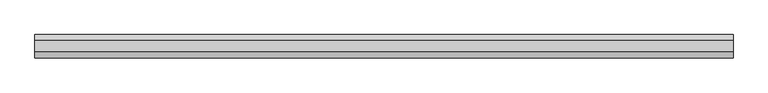
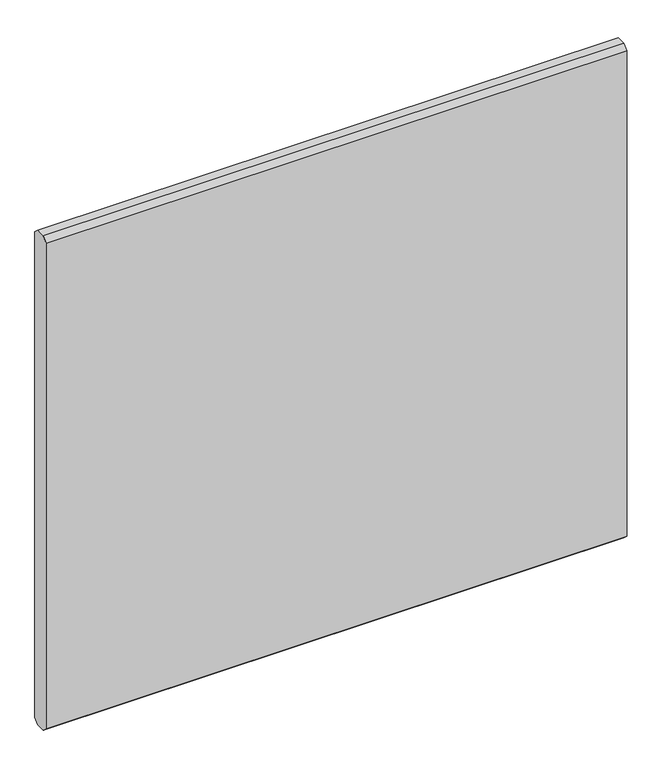
"""IFC4 building model written with IfcOpenShell, lengths in millimetres: proxy geometry, .RIPA : RIPA."""

from ifc_helpers import new_model, si_unit, frame, origin, place, context, project, spatial, polyline, outline, extrude, source, transform, mapped, element, save


def generic_models_0c544f32(model_context):
    return source(origin(), model_context, "Body", "SweptSolid", [
        extrude(outline(polyline([(-12.5, 1350.0), (12.5, 1350.0), (25.0, 1337.5), (25.0, 12.5), (12.5, 0.0), (-12.5, 0.0), (-25.0, 12.5), (-25.0, 1337.5), (-12.5, 1350.0)])), frame((-750.0, 0.0, 0.0), z_axis=(1.0, 0.0, 0.0), x_axis=(0.0, 1.0, 0.0)), (0.0, 0.0, 1.0), 1500.0),
    ])


if __name__ == "__main__":
    model = new_model("IFC4")
    model_context = context("Model", 3, world=origin())
    ifc_project = project(units=[si_unit("LENGTHUNIT", "METRE", prefix="MILLI")], contexts=[model_context])
    site = spatial("IfcSite", under=ifc_project)
    building = spatial("IfcBuilding", under=site)
    placement = place(None, origin())
    generic_models_shape = generic_models_0c544f32(model_context)
    element("IfcBuildingElementProxy", 1, Name=".RIPA : RIPA", ObjectType=".RIPA : RIPA", at=placement, inside=building, context=model_context, shape_type="MappedRepresentation", body=[
        mapped(generic_models_shape, transform((0.0, 0.0, 0.0), x_axis=(1.0, 0.0, 0.0), y_axis=(0.0, 1.0, 0.0), z_axis=(0.0, 0.0, 1.0))),
    ])
    save(model, "model.ifc")

# Revit data of these elements
# Type ".RIPA : RIPA"
#   Ripa_largura [instance default] = 0.30 m
#   Ripa_espessura [instance default] = 0.025 m
#   Ripa_comprimento [instance default] = 0.80 m
#   Ripa_chanfo [instance default] = 0.00625 m
#   Ripa_material [instance default] = none
# Element 1 (IfcBuildingElementProxy, ".RIPA : RIPA")
#   Ripa_largura = 1.35 m
#   Ripa_espessura = 0.05 m
#   Ripa_comprimento = 1.50 m
#   Ripa_chanfo = 0.0125 m
#   Ripa_material = .MADEIRA_CEREJEIRA CLARO
#   Materials on its faces: ".MADEIRA_CEREJEIRA CLARO"
# Materials
#   ".MADEIRA_CEREJEIRA CLARO": class ".CC_MADEIRA REVEST.", colour RGB 233 182 144, transparency 0, Cost = 0
